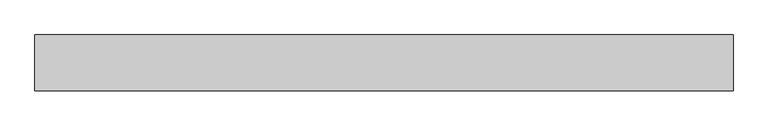
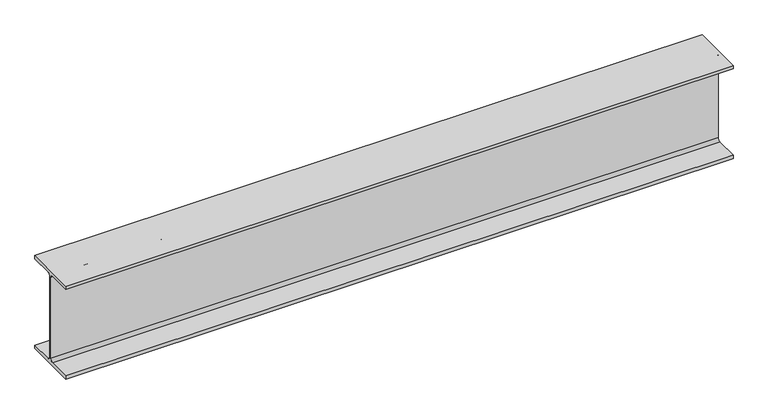
"""IFC4 building model written with IfcOpenShell, lengths in millimetres: beam geometry, Steel Beam_H-KSD3502 : H_SB_ASB_H-194x150x6x9."""

from ifc_helpers import new_model, si_unit, point, frame, frame_2d, origin, place, context, project, spatial, polyline, circle_curve, trimmed, segment, composite_curve, outline, extrude, source, transform, mapped, element, save


def beam_6061688a(model_context):
    return source(origin(), model_context, "Body", "SweptSolid", [
        extrude(outline(composite_curve([segment(polyline([(-82.5, -141.5), (-11.9, -141.5)]), True, "CONTINUOUS"), segment(trimmed(circle_curve(frame_2d((-11.9, -132.6)), 8.9), [point((-11.9, -141.5))], [point((-3.0, -132.6))], True, "CARTESIAN"), True, "CONTINUOUS"), segment(polyline([(-3.0, -132.6), (-3.0, 132.6)]), True, "CONTINUOUS"), segment(trimmed(circle_curve(frame_2d((-11.9, 132.6)), 8.9), [point((-3.0, 132.6))], [point((-11.9, 141.5))], True, "CARTESIAN"), True, "CONTINUOUS"), segment(polyline([(-11.9, 141.5), (-82.5, 141.5), (-82.5, 151.7), (82.5, 151.7), (82.5, 141.5), (11.9, 141.5)]), True, "CONTINUOUS"), segment(trimmed(circle_curve(frame_2d((11.9, 132.6)), 8.9), [point((11.9, 141.5))], [point((3.0, 132.6))], True, "CARTESIAN"), True, "CONTINUOUS"), segment(polyline([(3.0, 132.6), (3.0, -132.6)]), True, "CONTINUOUS"), segment(trimmed(circle_curve(frame_2d((11.9, -132.6)), 8.9), [point((3.0, -132.6))], [point((11.9, -141.5))], True, "CARTESIAN"), True, "CONTINUOUS"), segment(polyline([(11.9, -141.5), (82.5, -141.5), (82.5, -151.7), (-82.5, -151.7), (-82.5, -141.5)]), True, "CONTINUOUS")], self_intersect=False)), frame((-1047.9231301, 0.0, 0.0), z_axis=(1.0, 0.0, 0.0), x_axis=(0.0, 1.0, 0.0)), (0.0, 0.0, 1.0), 2060.1030758),
    ])


if __name__ == "__main__":
    model = new_model("IFC4")
    model_context = context("Model", 3, world=origin())
    ifc_project = project(units=[si_unit("LENGTHUNIT", "METRE", prefix="MILLI")], contexts=[model_context])
    site = spatial("IfcSite", under=ifc_project)
    building = spatial("IfcBuilding", under=site)
    placement = place(None, origin())
    beam_shape = beam_6061688a(model_context)
    element("IfcBeam", 1, ObjectType="Steel Beam_H-KSD3502 : H_SB_ASB_H-194x150x6x9", at=placement, inside=building, context=model_context, shape_type="MappedRepresentation", body=[
        mapped(beam_shape, transform((0.0, 0.0, 0.0), x_axis=(1.0, 0.0, 0.0), y_axis=(0.0, 1.0, 0.0), z_axis=(0.0, 0.0, 1.0))),
    ])
    save(model, "model.ifc")

# Revit data of these elements
# Type "Steel Beam_H-KSD3502 : H_SB_ASB_H-194x150x6x9"
#   Width = 15.0 cm
#   Web Thickness = 0.6 cm
#   Web Fillet = 1.3 cm
#   Warping Constant = 43316.0 cm⁶
#   Torsional Moment of Inertia = 8.622 cm⁴
#   Torsional Modulus = 1.0 cm³
#   Section Area = 39.01 cm²
#   Plastic Modulus weak axis = 104.0 cm³
#   Plastic Modulus strong axis = 309.0 cm³
#   Perimeter = 0.95 m²/m
#   Nominal Weight = 30.60 kgf/m
#   Moment of Inertia weak axis = 507.00 cm⁴
#   Moment of Inertia strong axis = 2690.00 cm⁴
#   Height = 19.4 cm
#   Flange Thickness = 0.9 cm
#   Elastic Modulus weak axis = 67.6 cm³
#   Elastic Modulus strong axis = 277.0 cm³
#   Centroid Vertical = 9.7 cm
#   Centroid Horizontal = 7.5 cm
#   Length [instance default] = 1.5240 m
#   Structural Material [instance default] = Steel, 45-345
#   Assembly Code = ""
# Element 1 (IfcBeam, "Steel Beam_H-KSD3502 : H_SB_ASB_H-194x150x6x9")
#   Structural Material = none
# Materials
#   "Steel, 45-345": class "Metal", colour RGB 189 187 185, transparency 0, Description = "Steel 345 MPa", Cost = 0
